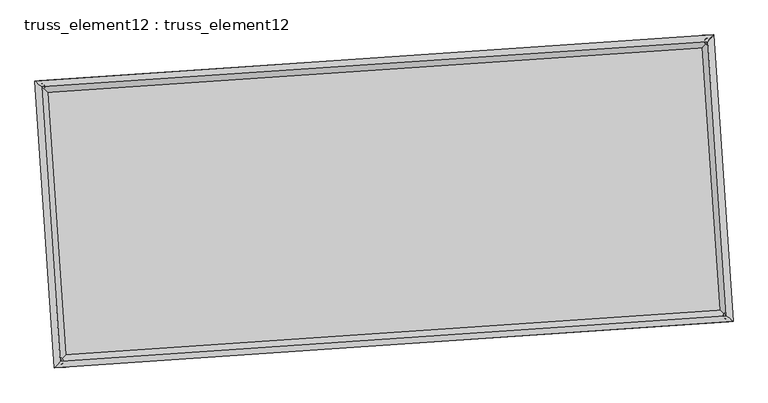
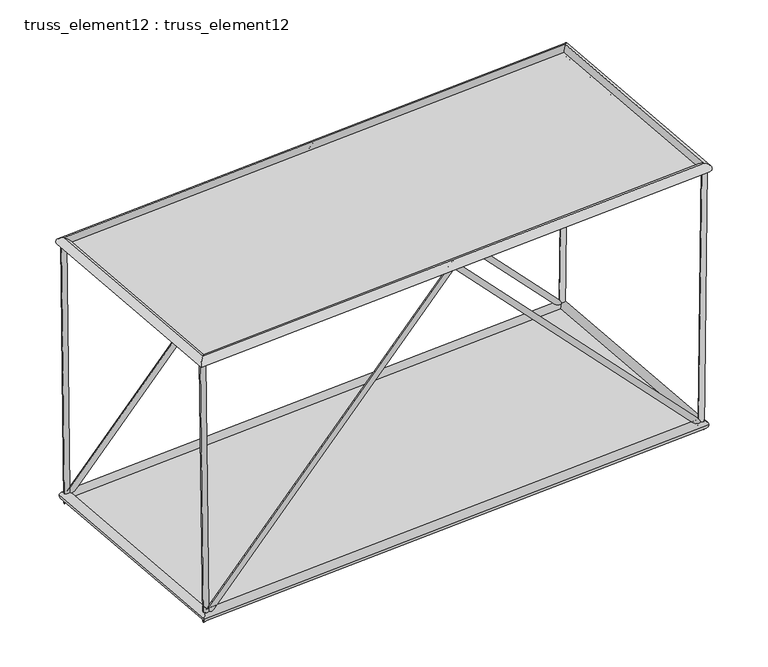
"""IFC4 building model written with IfcOpenShell, lengths in millimetres: plate geometry, truss_element12 : truss_element12."""

import ifcopenshell
import ifcopenshell.guid

model = None  # the IFC model being written
_history = None  # IfcOwnerHistory: only IFC2X3 demands one
_inside = {}  # id of a spatial element -> (the spatial element, [elements in it])
_under = {}  # id of a project, library or spatial element -> (it, [spatial elements below it])
_declared = {}  # id of a project -> (the project, [libraries it declares])
_typed = {}  # id of a type object -> (the type object, [elements of that type])
_made_of = {}  # id of a material, layer set ... -> (it, [elements and type objects made of it])


def new_model(schema):
    """Start an empty IFC model of exactly this schema.

    Asked for "IFC4X3", IfcOpenShell would pick the latest addendum, in which some entities
    have other attributes; the version numbers below select the first issue.
    IFC2X3 requires an IfcOwnerHistory on every rooted entity: one is made here for all.
    """
    global model, _history
    if schema == "IFC4X3":
        model = ifcopenshell.file(schema_version=(4, 3, 0, 0))
    else:
        model = ifcopenshell.file(schema=schema)
    _inside.clear()
    _under.clear()
    _declared.clear()
    _typed.clear()
    _made_of.clear()
    _history = None
    if model.schema == "IFC2X3":
        org = make("IfcOrganization", Name="unknown")
        user = make(
            "IfcPersonAndOrganization",
            ThePerson=make("IfcPerson", FamilyName="unknown"),
            TheOrganization=org,
        )
        app = make(
            "IfcApplication",
            ApplicationDeveloper=org,
            Version="unknown",
            ApplicationFullName="unknown",
            ApplicationIdentifier="unknown",
        )
        _history = make(
            "IfcOwnerHistory",
            OwningUser=user,
            OwningApplication=app,
            ChangeAction="ADDED",
            CreationDate=0,
        )
    return model


def make(cls, **values):
    """One entity of the class cls with the attributes given. An attribute that is None is left unset."""
    return model.create_entity(
        cls, **{name: value for name, value in values.items() if value is not None}
    )


def rooted(cls, **values):
    """An entity with a GlobalId (a new one), such as an element, a storey or a relation."""
    return make(cls, GlobalId=ifcopenshell.guid.new(), OwnerHistory=_history, **values)


def si_unit(unit_type, name, prefix=None):
    """IfcSIUnit, for example si_unit("LENGTHUNIT", "METRE", prefix="MILLI")."""
    return make("IfcSIUnit", UnitType=unit_type, Prefix=prefix, Name=name)


def assignment(units):
    """IfcUnitAssignment: the units of a project."""
    return None if units is None else make("IfcUnitAssignment", Units=units)


def point(xyz):
    """IfcCartesianPoint."""
    return None if xyz is None else make("IfcCartesianPoint", Coordinates=xyz)


def direction(xyz):
    """IfcDirection."""
    return None if xyz is None else make("IfcDirection", DirectionRatios=xyz)


def frame(location, z_axis=None, x_axis=None):
    """IfcAxis2Placement3D, a coordinate frame: its origin and axes. An axis left out is left unset."""
    return make(
        "IfcAxis2Placement3D",
        Location=point(location),
        Axis=direction(z_axis),
        RefDirection=direction(x_axis),
    )


def origin():
    """The frame at (0, 0, 0) with its axes left unset."""
    return frame((0.0, 0.0, 0.0))


def origin_with_axes():
    """The frame at (0, 0, 0) with the z axis (0, 0, 1) and the x axis (1, 0, 0) written out."""
    return frame((0.0, 0.0, 0.0), z_axis=(0.0, 0.0, 1.0), x_axis=(1.0, 0.0, 0.0))


def place(relative_to, where):
    """IfcLocalPlacement: puts the frame where relative to a parent placement (None: the world)."""
    return make(
        "IfcLocalPlacement", PlacementRelTo=relative_to, RelativePlacement=where
    )


def context(
    kind, dimensions, precision=None, world=None, true_north=None, identifier=None
):
    """IfcGeometricRepresentationContext, for example the 3D "Model" context."""
    return make(
        "IfcGeometricRepresentationContext",
        ContextIdentifier=identifier,
        ContextType=kind,
        CoordinateSpaceDimension=dimensions,
        Precision=precision,
        WorldCoordinateSystem=world,
        TrueNorth=true_north,
    )


def project(units=None, contexts=None):
    """IfcProject with its units and contexts."""
    return rooted(
        "IfcProject",
        Name="project",
        RepresentationContexts=contexts,
        UnitsInContext=assignment(units),
    )


def spatial(cls, under=None, at=None, **own):
    """A site, building, storey or space (cls), placed at a placement, below another one or the project."""
    s = rooted(cls, ObjectPlacement=at, **own)
    if under is not None:
        _under.setdefault(under.id(), (under, []))[1].append(s)
    return s


def polyline(points):
    """IfcPolyline through the points."""
    return make("IfcPolyline", Points=[point(p) for p in points])


def circle_curve(where, radius):
    """IfcCircle in the frame where."""
    return make("IfcCircle", Position=where, Radius=radius)


def ellipse_curve(where, semi_axis1, semi_axis2):
    """IfcEllipse in the frame where."""
    return make(
        "IfcEllipse", Position=where, SemiAxis1=semi_axis1, SemiAxis2=semi_axis2
    )


def outline(outer, holes=None, kind="AREA"):
    """IfcArbitraryClosedProfileDef: a profile drawn as a closed curve; with holes, ...WithVoids."""
    if holes is None:
        return make("IfcArbitraryClosedProfileDef", ProfileType=kind, OuterCurve=outer)
    return make(
        "IfcArbitraryProfileDefWithVoids",
        ProfileType=kind,
        OuterCurve=outer,
        InnerCurves=holes,
    )


def extrude(swept, where, along, depth):
    """IfcExtrudedAreaSolid: the profile swept, set in the frame where, extruded along a direction by depth."""
    return make(
        "IfcExtrudedAreaSolid",
        SweptArea=swept,
        Position=where,
        ExtrudedDirection=direction(along),
        Depth=depth,
    )


def shape(context_of_items, identifier, shape_type, items):
    """IfcShapeRepresentation: the items that make up one representation, for example the "Body"."""
    return make(
        "IfcShapeRepresentation",
        ContextOfItems=context_of_items,
        RepresentationIdentifier=identifier,
        RepresentationType=shape_type,
        Items=items,
    )


def source(mapping_origin, context_of_items, identifier, shape_type, items):
    """IfcRepresentationMap: a shape defined once, which mapped items show again and again."""
    return make(
        "IfcRepresentationMap",
        MappingOrigin=mapping_origin,
        MappedRepresentation=shape(context_of_items, identifier, shape_type, items),
    )


def transform(
    local_origin,
    x_axis=None,
    y_axis=None,
    z_axis=None,
    scale=None,
    scale2=None,
    scale3=None,
    uniform=True,
):
    """IfcCartesianTransformationOperator3D, or its non-uniform kind. x_axis, y_axis, z_axis: its Axis1, 2, 3."""
    if uniform:
        return make(
            "IfcCartesianTransformationOperator3D",
            Axis1=direction(x_axis),
            Axis2=direction(y_axis),
            LocalOrigin=point(local_origin),
            Scale=scale,
            Axis3=direction(z_axis),
        )
    return make(
        "IfcCartesianTransformationOperator3DnonUniform",
        Axis1=direction(x_axis),
        Axis2=direction(y_axis),
        LocalOrigin=point(local_origin),
        Scale=scale,
        Axis3=direction(z_axis),
        Scale2=scale2,
        Scale3=scale3,
    )


def mapped(mapping_source, mapping_target):
    """IfcMappedItem: shows the shape of a source again, moved by a transform."""
    return make(
        "IfcMappedItem", MappingSource=mapping_source, MappingTarget=mapping_target
    )


def made_of(thing, what):
    """Note that an element or type object is made of a material, layer set ...; save() writes the relation."""
    if what is not None:
        _made_of.setdefault(what.id(), (what, []))[1].append(thing)
    return thing


def element(
    cls,
    number,
    at=None,
    inside=None,
    cuts=None,
    type_object=None,
    material=None,
    context=None,
    identifier="Body",
    shape_type=None,
    held_by="IfcProductDefinitionShape",
    body=None,
    shapes=None,
    **own,
):
    """One element of the class cls, such as IfcWall. Its Tag is "e" and its number.

    at: its placement. inside: the storey or other place that contains it. cuts: it is an
    opening in that element (IfcRelVoidsElement). A single representation is given by context,
    identifier, shape_type and body (its items); several are given by shapes. held_by: the class
    of the entity that holds the representations. save() writes the other relations.
    """
    e = rooted(cls, Tag="e%d" % number, ObjectPlacement=at, **own)
    if body is not None:
        shapes = [shape(context, identifier, shape_type, body)]
    if shapes is not None:
        e.Representation = make(held_by, Representations=shapes)
    if inside is not None:
        _inside.setdefault(inside.id(), (inside, []))[1].append(e)
    if cuts is not None:
        rooted(
            "IfcRelVoidsElement", RelatingBuildingElement=cuts, RelatedOpeningElement=e
        )
    if type_object is not None:
        _typed.setdefault(type_object.id(), (type_object, []))[1].append(e)
    return made_of(e, material)


def aggregate(whole, parts):
    """IfcRelAggregates: a whole, such as a stair, and the parts it consists of."""
    return rooted("IfcRelAggregates", RelatingObject=whole, RelatedObjects=parts)


def save(model, path):
    """Write the relations noted so far, then the file.

    IfcRelAggregates (storeys below a building ...), IfcRelContainedInSpatialStructure (elements
    in a storey), IfcRelDefinesByType, IfcRelAssociatesMaterial and IfcRelDeclares: one each for
    every whole, place, type object, material and project.
    """
    for whole, parts in _under.values():
        aggregate(whole, parts)
    for where, things in _inside.values():
        rooted(
            "IfcRelContainedInSpatialStructure",
            RelatedElements=things,
            RelatingStructure=where,
        )
    for kind, things in _typed.values():
        rooted("IfcRelDefinesByType", RelatedObjects=things, RelatingType=kind)
    for what, things in _made_of.values():
        rooted("IfcRelAssociatesMaterial", RelatedObjects=things, RelatingMaterial=what)
    for by, libraries in _declared.values():
        rooted("IfcRelDeclares", RelatingContext=by, RelatedDefinitions=libraries)
    model.write(path)


def plane_surface(at):
    """IfcPlane: the flat surface through the origin of the frame at, square to its z axis."""
    return make("IfcPlane", Position=at)


def cylinder_surface(at, radius):
    """IfcCylindricalSurface: all points at the distance radius from the z axis of the frame at."""
    return make("IfcCylindricalSurface", Position=at, Radius=radius)


def advanced_brep(points, edges, surfaces, faces):
    """IfcAdvancedBrep: a solid bounded by faces that lie on surfaces and meet in shared edges.

    An edge is (start, end): straight between two places in points (the first is 0);
    or (start, end, curve); or (start, end, curve, False) where it runs against its curve.
    A face is (place in surfaces, loops), or (place, loops, False) where it looks against
    its surface's normal. A loop lists edges by number (the first is 1), with a minus sign
    where the edge is run from its end to its start. The first loop is the outer one.
    """
    corners = [point(p) for p in points]
    vertices = [make("IfcVertexPoint", VertexGeometry=c) for c in corners]
    made = []
    for start, end, *more in edges:
        made.append(
            make(
                "IfcEdgeCurve",
                EdgeStart=vertices[start],
                EdgeEnd=vertices[end],
                EdgeGeometry=more[0] if more else make("IfcPolyline", Points=[corners[start], corners[end]]),
                SameSense=more[1] if len(more) > 1 else True,
            )
        )
    hull = []
    for where, loops, *sense in faces:
        bounds = []
        for j, loop in enumerate(loops):
            ring = [make("IfcOrientedEdge", EdgeElement=made[abs(k) - 1], Orientation=k > 0) for k in loop]
            bounds.append(
                make(
                    "IfcFaceOuterBound" if j == 0 else "IfcFaceBound",
                    Bound=make("IfcEdgeLoop", EdgeList=ring),
                    Orientation=True,
                )
            )
        hull.append(make("IfcAdvancedFace", Bounds=bounds, FaceSurface=surfaces[where], SameSense=sense[0] if sense else True))
    return make("IfcAdvancedBrep", Outer=make("IfcClosedShell", CfsFaces=hull))


def truss_element12_truss_element12_8f72c4cc(model_context):
    return source(origin(), model_context, "Body", "SolidModel", [
        advanced_brep(
        [(-3727.2192532, 2271.9774942, 5000.2332074), (-3826.3148624, 2258.6167835, 4998.9875555), (-3666.4649033, 2276.1201024, 122.5964802), (-3762.5219795, 2262.9665777, -122.5964802), (1064.2915004, 2598.6923983, 5071.7241835), (1064.7311595, 2592.1186192, 4927.4822392), (5793.9313565, 2921.188561, 122.5885273), (5890.8296205, 2921.1919275, -122.5885273), (5855.7938545, 2925.4067296, 5000.230225), (5955.7855808, 2925.6210275, 4998.9618575)],
        [
            (0, 1, circle_curve(frame((-3776.7670578, 2265.2971389, 4999.6103815), z_axis=(-0.012454723282468943, -0.0008492402357976954, 0.9999220762934375), x_axis=(-0.1336072742715059, 0.9910340154549612, -0.0008224797592794459)), 50.0)),
            (1, 0, circle_curve(frame((-3776.7670578, 2265.2971389, 4999.6103815), z_axis=(-0.012454723282468943, -0.0008492402357976954, 0.9999220762934375), x_axis=(-0.1336072742715059, 0.9910340154549612, -0.0008224797592794459)), 50.0)),
            (0, 2),
            (2, 3, ellipse_curve(frame((-3714.4934414, 2269.54334, 0.0), z_axis=(-0.9280745157714434, -0.06328187328893568, 0.36697833408614733), x_axis=(0.3661281906369683, 0.02496488953598211, 0.9302294890570586)), 132.0786249, 50.0)),
            (3, 1),
            (3, 2, ellipse_curve(frame((-3714.4934414, 2269.54334, 0.0), z_axis=(-0.9280745157714434, -0.06328187328893568, 0.36697833408614733), x_axis=(0.3661281906369683, 0.02496488953598211, 0.9302294890570586)), 132.0786249, 50.0)),
            (2, 4),
            (4, 5, ellipse_curve(frame((1064.5113299, 2595.4055087, 4999.6032114), z_axis=(-0.9976833943172301, -0.06802823810885233, 5.935870352728737e-05), x_axis=(-5.9221192921833396e-05, -4.03806802274625e-06, -0.9999999982382721)), 72.2780144, 50.0)),
            (5, 3),
            (5, 4, ellipse_curve(frame((1064.5113299, 2595.4055087, 4999.6032114), z_axis=(-0.9976833943172301, -0.06802823810885233, 5.935870352728737e-05), x_axis=(-5.9221192921833396e-05, -4.03806802274625e-06, -0.9999999982382721)), 72.2780144, 50.0)),
            (4, 6),
            (6, 7, ellipse_curve(frame((5842.3804885, 2921.1902443, 0.0), z_axis=(-0.9281379125811653, -0.06328619607639555, -0.36681721962805564), x_axis=(-0.3659674494172622, -0.024953929203248196, 0.9302930330730972)), 132.0610358, 50.0)),
            (7, 5),
            (7, 6, ellipse_curve(frame((5842.3804885, 2921.1902443, 0.0), z_axis=(-0.9281379125811653, -0.06328619607639555, -0.36681721962805564), x_axis=(-0.3659674494172622, -0.024953929203248196, 0.9302930330730972)), 132.0610358, 50.0)),
            (8, 9, circle_curve(frame((5905.7897177, 2925.5138785, 4999.5960413), z_axis=(0.012681845830496502, 0.0008647268589705681, 0.9999192082532424), x_axis=(-0.0021537739507081696, 0.9999973299402997, -0.0008374783822429829)), 50.0)),
            (9, 8, circle_curve(frame((5905.7897177, 2925.5138785, 4999.5960413), z_axis=(0.012681845830496502, 0.0008647268589705681, 0.9999192082532424), x_axis=(-0.0021537739507081696, 0.9999973299402997, -0.0008374783822429829)), 50.0)),
            (6, 8),
            (9, 7),
        ],
        [
            plane_surface(frame((-3776.7670578, 2315.2971208, 4999.6528468), z_axis=(-0.012454723282470215, -0.0008492402357928436, 0.9999220762934375), x_axis=(0.9999224369259634, -1.0577872589401237e-05, 0.012454718790543492))),
            cylinder_surface(frame((-3776.7670578, 2265.2971389, 4999.6103815), z_axis=(-0.012454723282468943, -0.0008492402357976954, 0.9999220762934375), x_axis=(-0.1336072742715059, 0.9910340154549612, -0.0008224797592794459)), 50.0),
            cylinder_surface(frame((-3714.4934414, 2269.54334, 0.0), z_axis=(-0.6902134913462219, -0.04706303422778228, -0.7220736854178621), x_axis=(-0.020417106549851006, 0.998752022715791, -0.04558002721859809)), 50.0),
            cylinder_surface(frame((1064.5113299, 2595.4055087, 4999.6032114), z_axis=(-0.6901279623524434, -0.04705720233082522, 0.7221558109494518), x_axis=(-0.11534915142313243, 0.9922789674463691, -0.045574379091006735)), 50.0),
            plane_surface(frame((5905.7897177, 2875.5138972, 4999.6392811), z_axis=(0.01268184583049596, 0.0008647268589738932, 0.9999192082532424), x_axis=(0.9999195821596514, -1.0967214670642978e-05, -0.012681841088291169))),
            cylinder_surface(frame((5842.3804885, 2921.1902443, 0.0), z_axis=(-0.012681845830496502, -0.0008647268589705681, -0.9999192082532424), x_axis=(-0.0021537739507081696, 0.9999973299402997, -0.0008374783822429829)), 50.0),
        ],
        [
            (0, [[1, 2]]),
            (1, [[-1, 3, 4, 5]]),
            (1, [[-2, -5, 6, -3]]),
            (2, [[-4, 7, 8, 9]]),
            (2, [[-6, -9, 10, -7]]),
            (3, [[-8, 11, 12, 13]]),
            (3, [[-10, -13, 14, -11]]),
            (4, [[15, 16]]),
            (5, [[-12, 17, -16, 18]]),
            (5, [[-14, -18, -15, -17]]),
        ],
    ),
        advanced_brep(
        [(-3455.1063003, -1718.7560901, 5000.2332074), (-3554.2019095, -1732.1168008, 4998.9875555), (-3394.3519504, -1714.6134819, 122.5964802), (-3490.4090266, -1727.7670066, -122.5964802), (1336.4044533, -1392.041186, 5071.7241835), (1336.8441124, -1398.6149651, 4927.4822392), (6066.0443094, -1069.5450233, 122.5885273), (6162.9425734, -1069.5416568, -122.5885273), (6127.9068074, -1065.3268547, 5000.230225), (6227.8985337, -1065.1125568, 4998.9618575)],
        [
            (0, 1, circle_curve(frame((-3504.6541049, -1725.4364454, 4999.6103815), z_axis=(-0.012454723282468884, -0.0008492402357977014, 0.9999220762934377), x_axis=(-0.13360727427150593, 0.9910340154549612, -0.0008224797592794322)), 50.0)),
            (1, 0, circle_curve(frame((-3504.6541049, -1725.4364454, 4999.6103815), z_axis=(-0.012454723282468884, -0.0008492402357977014, 0.9999220762934377), x_axis=(-0.13360727427150593, 0.9910340154549612, -0.0008224797592794322)), 50.0)),
            (0, 2),
            (2, 3, ellipse_curve(frame((-3442.3804885, -1721.1902443, 0.0), z_axis=(-0.9280745157714434, -0.06328187328893571, 0.3669783340861473), x_axis=(0.36612819063696816, 0.024964889535982103, 0.9302294890570585)), 132.0786249, 50.0)),
            (3, 1),
            (3, 2, ellipse_curve(frame((-3442.3804885, -1721.1902443, 0.0), z_axis=(-0.9280745157714434, -0.06328187328893571, 0.3669783340861473), x_axis=(0.36612819063696816, 0.024964889535982103, 0.9302294890570585)), 132.0786249, 50.0)),
            (2, 4),
            (4, 5, ellipse_curve(frame((1336.6242828, -1395.3280756, 4999.6032114), z_axis=(-0.9976833943172301, -0.0680282381088523, 5.9358703526404644e-05), x_axis=(-5.9221192920910944e-05, -4.0380680227270335e-06, -0.9999999982382721)), 72.2780144, 50.0)),
            (5, 3),
            (5, 4, ellipse_curve(frame((1336.6242828, -1395.3280756, 4999.6032114), z_axis=(-0.9976833943172301, -0.0680282381088523, 5.9358703526404644e-05), x_axis=(-5.9221192920910944e-05, -4.0380680227270335e-06, -0.9999999982382721)), 72.2780144, 50.0)),
            (4, 6),
            (6, 7, ellipse_curve(frame((6114.4934414, -1069.54334, 0.0), z_axis=(-0.9281379125811651, -0.06328619607639552, -0.36681721962805613), x_axis=(-0.3659674494172627, -0.024953929203248182, 0.9302930330730971)), 132.0610358, 50.0)),
            (7, 5),
            (7, 6, ellipse_curve(frame((6114.4934414, -1069.54334, 0.0), z_axis=(-0.9281379125811651, -0.06328619607639552, -0.36681721962805613), x_axis=(-0.3659674494172627, -0.024953929203248182, 0.9302930330730971)), 132.0610358, 50.0)),
            (8, 9, circle_curve(frame((6177.9026706, -1065.2197058, 4999.5960413), z_axis=(0.01268184583049621, 0.0008647268589706002, 0.9999192082532423), x_axis=(-0.002153773950708037, 0.9999973299402997, -0.0008374783822430173)), 50.0)),
            (9, 8, circle_curve(frame((6177.9026706, -1065.2197058, 4999.5960413), z_axis=(0.01268184583049621, 0.0008647268589706002, 0.9999192082532423), x_axis=(-0.002153773950708037, 0.9999973299402997, -0.0008374783822430173)), 50.0)),
            (6, 8),
            (9, 7),
        ],
        [
            plane_surface(frame((-3504.6541049, -1675.4364635, 4999.6528468), z_axis=(-0.012454723282470215, -0.0008492402357928367, 0.9999220762934375), x_axis=(0.9999224369259634, -1.0577872589401237e-05, 0.012454718790543492))),
            cylinder_surface(frame((-3504.6541049, -1725.4364454, 4999.6103815), z_axis=(-0.012454723282468884, -0.0008492402357977014, 0.9999220762934377), x_axis=(-0.13360727427150593, 0.9910340154549612, -0.0008224797592794322)), 50.0),
            cylinder_surface(frame((-3442.3804885, -1721.1902443, 0.0), z_axis=(-0.6902134913462216, -0.04706303422778227, -0.7220736854178624), x_axis=(-0.020417106549850947, 0.998752022715791, -0.04558002721859812)), 50.0),
            cylinder_surface(frame((1336.6242828, -1395.3280756, 4999.6032114), z_axis=(-0.6901279623524446, -0.04705720233082525, 0.722155810949451), x_axis=(-0.11534915142313235, 0.9922789674463693, -0.04557437909100684)), 50.0),
            plane_surface(frame((6177.9026706, -1115.2196871, 4999.6392811), z_axis=(0.01268184583049596, 0.0008647268589738886, 0.9999192082532424), x_axis=(0.9999195821596514, -1.0967214670642978e-05, -0.012681841088291169))),
            cylinder_surface(frame((6114.4934414, -1069.54334, 0.0), z_axis=(-0.01268184583049621, -0.0008647268589706002, -0.9999192082532423), x_axis=(-0.002153773950708037, 0.9999973299402997, -0.0008374783822430173)), 50.0),
        ],
        [
            (0, [[1, 2]]),
            (1, [[-1, 3, 4, 5]]),
            (1, [[-2, -5, 6, -3]]),
            (2, [[-4, 7, 8, 9]]),
            (2, [[-6, -9, 10, -7]]),
            (3, [[-8, 11, 12, 13]]),
            (3, [[-10, -13, 14, -11]]),
            (4, [[15, 16]]),
            (5, [[-12, 17, -16, 18]]),
            (5, [[-14, -18, -15, -17]]),
        ],
    ),
        advanced_brep(
        [(-3504.657868, -1725.4406162, 4909.6103816), (-3504.6503418, -1725.4322746, 5089.6103814), (-3776.7627634, 2265.2935175, 5089.6103814), (-3776.7713523, 2265.3007603, 4909.6103816), (5905.7862199, 2925.5097258, 5089.5960412), (5905.7932154, 2925.5180313, 4909.5960413), (6177.8986415, -1065.2160663, 5089.5960412), (6177.9066997, -1065.2233452, 4909.5960413)],
        [
            (0, 1, ellipse_curve(frame((-3504.6541049, -1725.4364454, 4999.6103815), z_axis=(-0.7535719234046849, 0.6573654662781367, 1.0448235056074835e-06), x_axis=(-0.6573654662773142, -0.7535719234054024, 1.0448234933563717e-06)), 127.2792206, 90.0)),
            (1, 2),
            (2, 3, ellipse_curve(frame((-3776.7670578, 2265.2971389, 4999.6103815), z_axis=(-0.6573654662773138, -0.7535719234054027, 1.0448234939876744e-06), x_axis=(0.753571923404685, -0.6573654662781364, -1.044823506238787e-06)), 127.2792206, 90.0)),
            (3, 0),
            (1, 0, ellipse_curve(frame((-3504.6541049, -1725.4364454, 4999.6103815), z_axis=(-0.7535719234046849, 0.6573654662781367, 1.0448235056074835e-06), x_axis=(-0.6573654662773142, -0.7535719234054024, 1.0448234933563717e-06)), 127.2792206, 90.0)),
            (3, 2, ellipse_curve(frame((-3776.7670578, 2265.2971389, 4999.6103815), z_axis=(-0.6573654662773138, -0.7535719234054027, 1.0448234939876744e-06), x_axis=(0.753571923404685, -0.6573654662781364, -1.044823506238787e-06)), 127.2792206, 90.0)),
            (2, 4),
            (4, 5, ellipse_curve(frame((5905.7897177, 2925.5138785, 4999.5960413), z_axis=(-0.7535719234046856, 0.657365466278136, 1.0448235047075032e-06), x_axis=(-0.6573654662773132, -0.7535719234054032, 1.0448234955189582e-06)), 127.2792206, 90.0)),
            (5, 3),
            (5, 4, ellipse_curve(frame((5905.7897177, 2925.5138785, 4999.5960413), z_axis=(-0.7535719234046856, 0.657365466278136, 1.0448235047075032e-06), x_axis=(-0.6573654662773132, -0.7535719234054032, 1.0448234955189582e-06)), 127.2792206, 90.0)),
            (4, 6),
            (6, 7, ellipse_curve(frame((6177.9026706, -1065.2197058, 4999.5960413), z_axis=(0.6573654662773132, 0.7535719234054032, -1.0448234948876552e-06), x_axis=(-0.7535719234046856, 0.6573654662781359, 1.0448235040762e-06)), 127.2792206, 90.0)),
            (7, 5),
            (7, 6, ellipse_curve(frame((6177.9026706, -1065.2197058, 4999.5960413), z_axis=(0.6573654662773132, 0.7535719234054032, -1.0448234948876552e-06), x_axis=(-0.7535719234046856, 0.6573654662781359, 1.0448235040762e-06)), 127.2792206, 90.0)),
            (6, 1),
            (0, 7),
        ],
        [
            cylinder_surface(frame((-3504.6541049, -1725.4364454, 4999.6103815), z_axis=(0.06802823822869772, -0.9976833960748768, 0.0), x_axis=(-0.9976833950706322, -0.06802823816022209, 4.4868174597883384e-05)), 90.0),
            cylinder_surface(frame((-3776.7670578, 2265.2971389, 4999.6103815), z_axis=(-0.997683396073788, -0.06802823822862193, 1.4776035641462583e-06), x_axis=(-0.06802823810069086, 0.9976833951400486, 4.339057104379111e-05)), 90.0),
            cylinder_surface(frame((5905.7897177, 2925.5138785, 4999.5960413), z_axis=(-0.06802823822869962, 0.9976833960748769, 0.0), x_axis=(0.9976833951985631, 0.06802823816894711, 4.1912967474538696e-05)), 90.0),
            cylinder_surface(frame((6177.9026706, -1065.2197058, 4999.5960413), z_axis=(0.9976833960737879, 0.06802823822862185, -1.4776035632534604e-06), x_axis=(0.06802823822862185, -0.9976833951313253, 4.339057102990407e-05)), 90.0),
        ],
        [
            (0, [[1, 2, 3, 4]]),
            (0, [[5, -4, 6, -2]]),
            (1, [[-3, 7, 8, 9]]),
            (1, [[-6, -9, 10, -7]]),
            (2, [[-8, 11, 12, 13]]),
            (2, [[-10, -13, 14, -11]]),
            (3, [[-12, 15, -1, 16]]),
            (3, [[-14, -16, -5, -15]]),
        ],
    ),
        advanced_brep(
        [(-3358.7115243, -1625.2761972, 0.0), (-3526.0494527, -1817.1042913, 0.0), (-3810.4074885, 2353.2123043, 0.0), (-3618.5793943, 2185.8743758, 0.0), (5926.0494527, 3017.1042913, 0.0), (5758.7115243, 2825.2761972, 0.0), (6210.4074885, -1153.2123043, 0.0), (6018.5793943, -985.8743758, 0.0)],
        [
            (0, 1, ellipse_curve(frame((-3442.3804885, -1721.1902443, 0.0), z_axis=(-0.7535719234054572, 0.6573654662780816, 0.0), x_axis=(-0.6573654662780816, -0.7535719234054573, 0.0)), 127.2792206, 90.0)),
            (1, 2),
            (2, 3, ellipse_curve(frame((-3714.4934414, 2269.54334, 0.0), z_axis=(-0.6573654662780816, -0.7535719234054573, 0.0), x_axis=(0.7535719234054572, -0.6573654662780816, 0.0)), 127.2792206, 90.0)),
            (3, 0),
            (1, 0, ellipse_curve(frame((-3442.3804885, -1721.1902443, 0.0), z_axis=(-0.7535719234054572, 0.6573654662780816, 0.0), x_axis=(-0.6573654662780816, -0.7535719234054573, 0.0)), 127.2792206, 90.0)),
            (3, 2, ellipse_curve(frame((-3714.4934414, 2269.54334, 0.0), z_axis=(-0.6573654662780816, -0.7535719234054573, 0.0), x_axis=(0.7535719234054572, -0.6573654662780816, 0.0)), 127.2792206, 90.0)),
            (2, 4),
            (4, 5, ellipse_curve(frame((5842.3804885, 2921.1902443, 0.0), z_axis=(-0.753571923405458, 0.6573654662780807, 0.0), x_axis=(-0.6573654662780808, -0.7535719234054579, 0.0)), 127.2792206, 90.0)),
            (5, 3),
            (5, 4, ellipse_curve(frame((5842.3804885, 2921.1902443, 0.0), z_axis=(-0.753571923405458, 0.6573654662780807, 0.0), x_axis=(-0.6573654662780808, -0.7535719234054579, 0.0)), 127.2792206, 90.0)),
            (4, 6),
            (6, 7, ellipse_curve(frame((6114.4934414, -1069.54334, 0.0), z_axis=(0.6573654662780809, 0.7535719234054579, 0.0), x_axis=(-0.753571923405458, 0.6573654662780809, 0.0)), 127.2792206, 90.0)),
            (7, 5),
            (7, 6, ellipse_curve(frame((6114.4934414, -1069.54334, 0.0), z_axis=(0.6573654662780809, 0.7535719234054579, 0.0), x_axis=(-0.753571923405458, 0.6573654662780809, 0.0)), 127.2792206, 90.0)),
            (6, 1),
            (0, 7),
        ],
        [
            cylinder_surface(frame((-3442.3804885, -1721.1902443, 0.0), z_axis=(0.06802823822870091, -0.9976833960748767, 0.0), x_axis=(-0.9976833960748767, -0.06802823822870091, 0.0)), 90.0),
            cylinder_surface(frame((-3714.4934414, 2269.54334, 0.0), z_axis=(-0.9976833960748768, -0.06802823822869955, 0.0), x_axis=(-0.06802823822869955, 0.9976833960748768, 0.0)), 90.0),
            cylinder_surface(frame((5842.3804885, 2921.1902443, 0.0), z_axis=(-0.06802823822870294, 0.9976833960748764, 0.0), x_axis=(0.9976833960748764, 0.06802823822870294, 0.0)), 90.0),
            cylinder_surface(frame((6114.4934414, -1069.54334, 0.0), z_axis=(0.9976833960748767, 0.06802823822869943, 0.0), x_axis=(0.06802823822869943, -0.9976833960748767, 0.0)), 90.0),
        ],
        [
            (0, [[1, 2, 3, 4]]),
            (0, [[5, -4, 6, -2]]),
            (1, [[-3, 7, 8, 9]]),
            (1, [[-6, -9, 10, -7]]),
            (2, [[-8, 11, 12, 13]]),
            (2, [[-10, -13, 14, -11]]),
            (3, [[-12, 15, -1, 16]]),
            (3, [[-14, -16, -5, -15]]),
        ],
    ),
        extrude(outline(polyline([(-3442.3804885, -1721.1902443), (-3714.4934414, 2269.54334), (5842.3804885, 2921.1902443), (6114.4934414, -1069.54334), (-3442.3804885, -1721.1902443)])), origin_with_axes(), (0.0, 0.0, 1.0), 20.0),
        extrude(outline(polyline([(-2000.0, 4852.5197541), (2000.0, 4852.5197541), (1999.9999999, -4852.5197541), (-2000.0000001, -4852.5197541), (-2000.0, 4852.5197541)])), frame((1200.5678064, 600.0387166, 4999.6032114), z_axis=(1.4741805425190185e-06, 1.005187586264448e-07, 0.9999999999989084), x_axis=(-0.06802823822870088, 0.9976833960748767, 0.0)), (0.0, 0.0, 1.0), 20.0),
    ])


if __name__ == "__main__":
    model = new_model("IFC4")
    model_context = context("Model", 3, world=origin())
    ifc_project = project(units=[si_unit("LENGTHUNIT", "METRE", prefix="MILLI")], contexts=[model_context])
    site = spatial("IfcSite", under=ifc_project)
    building = spatial("IfcBuilding", under=site)
    placement = place(None, origin())
    truss_element12_truss_element12_shape = truss_element12_truss_element12_8f72c4cc(model_context)
    element("IfcPlate", 1, ObjectType="truss_element12 : truss_element12", at=placement, inside=building, context=model_context, shape_type="MappedRepresentation", body=[
        mapped(truss_element12_truss_element12_shape, transform((0.0, 0.0, 0.0), x_axis=(1.0, 0.0, 0.0), y_axis=(0.0, 1.0, 0.0), z_axis=(0.0, 0.0, 1.0))),
    ])
    save(model, "model.ifc")

# Revit data of these elements
# Type "truss_element12 : truss_element12"
#   steellbar1 = 90 mm
#   steelbar2 = 50 mm
#   offset1 = 5000 mm
#   M = Default Roof
# Element 1 (IfcPlate, "truss_element12 : truss_element12")
#   Materials on its faces: "Default Roof"
# Materials
#   "Default Roof": class "Miscellaneous", colour RGB 0 127 0, transparency 0, Comments = "Rendering appearance not upgraded Rendering appearance not upgraded ", Cost = 0
